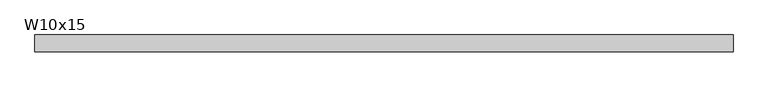
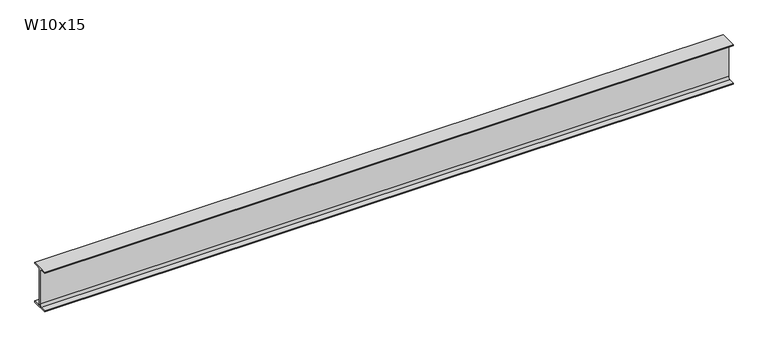
"""IFC4 building model written with IfcOpenShell, lengths in millimetres: beam geometry, RME W-Wide Flange : W10x15."""

from ifc_helpers import new_model, si_unit, point, frame, frame_2d, origin, place, context, project, spatial, polyline, circle_curve, trimmed, segment, composite_curve, outline, extrude, source, transform, mapped, element, save


def w10x15_17ba8876(model_context):
    return source(origin(), model_context, "Body", "SweptSolid", [
        extrude(outline(composite_curve([segment(polyline([(50.8, -120.142), (50.8, -127.0), (-50.8, -127.0), (-50.8, -120.142), (-16.7005, -120.142)]), True, "CONTINUOUS"), segment(trimmed(circle_curve(frame_2d((-16.7005, -106.3625)), 13.7795), [point((-16.7005, -120.142))], [point((-2.921, -106.3625))], True, "CARTESIAN"), True, "CONTINUOUS"), segment(polyline([(-2.921, -106.3625), (-2.921, 106.3625)]), True, "CONTINUOUS"), segment(trimmed(circle_curve(frame_2d((-16.7005, 106.3625)), 13.7795), [point((-2.921, 106.3625))], [point((-16.7005, 120.142))], True, "CARTESIAN"), True, "CONTINUOUS"), segment(polyline([(-16.7005, 120.142), (-50.8, 120.142), (-50.8, 127.0), (50.8, 127.0), (50.8, 120.142), (16.7005, 120.142)]), True, "CONTINUOUS"), segment(trimmed(circle_curve(frame_2d((16.7005, 106.3625)), 13.7795), [point((16.7005, 120.142))], [point((2.921, 106.3625))], True, "CARTESIAN"), True, "CONTINUOUS"), segment(polyline([(2.921, 106.3625), (2.921, -106.3625)]), True, "CONTINUOUS"), segment(trimmed(circle_curve(frame_2d((16.7005, -106.3625)), 13.7795), [point((2.921, -106.3625))], [point((16.7005, -120.142))], True, "CARTESIAN"), True, "CONTINUOUS"), segment(polyline([(16.7005, -120.142), (50.8, -120.142)]), True, "CONTINUOUS")], self_intersect=False)), frame((-2055.1406126, 0.0, 0.0), z_axis=(1.0, 0.0, 0.0), x_axis=(0.0, 1.0, 0.0)), (0.0, 0.0, 1.0), 4176.0406126),
    ])


if __name__ == "__main__":
    model = new_model("IFC4")
    model_context = context("Model", 3, world=origin())
    ifc_project = project(units=[si_unit("LENGTHUNIT", "METRE", prefix="MILLI")], contexts=[model_context])
    site = spatial("IfcSite", under=ifc_project)
    building = spatial("IfcBuilding", under=site)
    placement = place(None, origin())
    w10x15_shape = w10x15_17ba8876(model_context)
    element("IfcBeam", 1, ObjectType="RME W-Wide Flange : W10x15", at=placement, inside=building, context=model_context, shape_type="MappedRepresentation", body=[
        mapped(w10x15_shape, transform((0.0, 0.0, 0.0), x_axis=(1.0, 0.0, 0.0), y_axis=(0.0, 1.0, 0.0), z_axis=(0.0, 0.0, 1.0))),
    ])
    save(model, "model.ifc")

# Revit data of these elements
# Type "RME W-Wide Flange : W10x15"
#   WELD P [instance default] = ""
#   WELD LE [instance default] = ""
#   WELD D [instance default] = ""
#   TOP SECTION SIZE [instance default] = ""
#   TOP SECTION LENGTH [instance default] = ""
#   REMARKS [instance default] = ""
#   REINF TYPE [instance default] = ""
#   Nominal Size = "W24"
#   End Bearing Capacity [instance default] = ""
#   BOT SECTION SIZE [instance default] = ""
#   BOT SECTION LENGTH [instance default] = ""
#   Assembly Code = "B10"
#   W = 15
#   Start Extension Calculation [instance default] = 10' - 0"
#   Start Extension [instance default] = -0' - 0 1/2"
#   End Extension Calculation [instance default] = 10' - 0"
#   End Extension [instance default] = -0' - 0 1/2"
#   Length [instance default] = 5' - 0"
#   bf = 0' - 4"
#   d = 0' - 10"
#   k = 0' - 0 13/16"
#   k2 = 0' - 0.5425"
#   tf = 0' - 0.27"
#   tw = 0' - 0.23"
#   A = 0.030625 SF
#   Structural Material [instance default] = Metal - Steel - ASTM A992
# Element 1 (IfcBeam, "RME W-Wide Flange : W10x15")
#   Length = 13' - 11"
#   Materials on its faces: "Metal - Steel - ASTM A992"
# Materials
#   "Metal - Steel - ASTM A992": class "Metal", colour RGB 255 128 0, transparency 0
